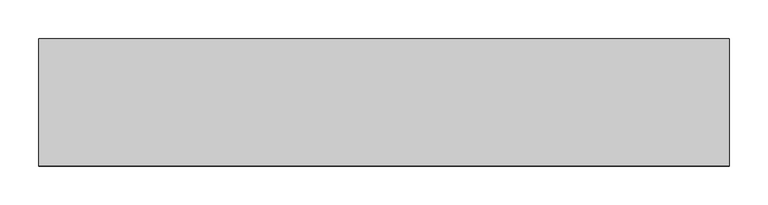
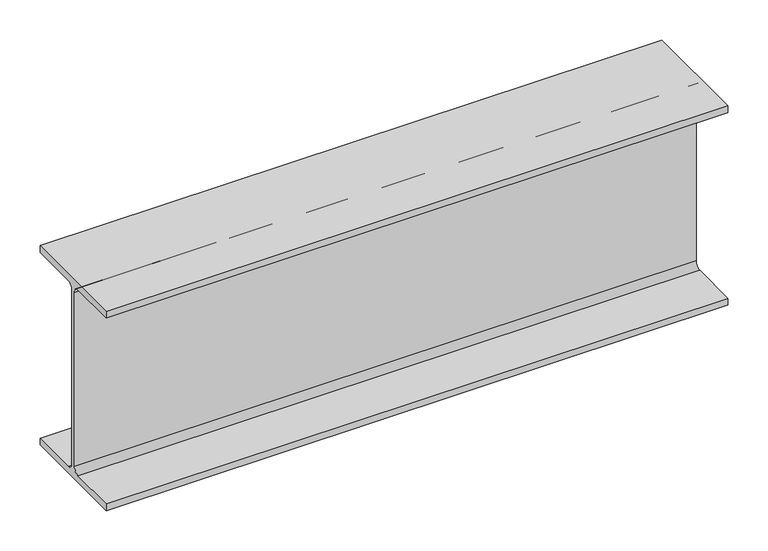
"""IFC4 building model written with IfcOpenShell, lengths in millimetres: beam geometry, Old_Steel Beam_H-KSD3502 : H_SB_ASB_H-300×150x6.5x9."""

import ifcopenshell
import ifcopenshell.guid

model = None  # the IFC model being written
_history = None  # IfcOwnerHistory: only IFC2X3 demands one
_inside = {}  # id of a spatial element -> (the spatial element, [elements in it])
_under = {}  # id of a project, library or spatial element -> (it, [spatial elements below it])
_declared = {}  # id of a project -> (the project, [libraries it declares])
_typed = {}  # id of a type object -> (the type object, [elements of that type])
_made_of = {}  # id of a material, layer set ... -> (it, [elements and type objects made of it])


def new_model(schema):
    """Start an empty IFC model of exactly this schema.

    Asked for "IFC4X3", IfcOpenShell would pick the latest addendum, in which some entities
    have other attributes; the version numbers below select the first issue.
    IFC2X3 requires an IfcOwnerHistory on every rooted entity: one is made here for all.
    """
    global model, _history
    if schema == "IFC4X3":
        model = ifcopenshell.file(schema_version=(4, 3, 0, 0))
    else:
        model = ifcopenshell.file(schema=schema)
    _inside.clear()
    _under.clear()
    _declared.clear()
    _typed.clear()
    _made_of.clear()
    _history = None
    if model.schema == "IFC2X3":
        org = make("IfcOrganization", Name="unknown")
        user = make(
            "IfcPersonAndOrganization",
            ThePerson=make("IfcPerson", FamilyName="unknown"),
            TheOrganization=org,
        )
        app = make(
            "IfcApplication",
            ApplicationDeveloper=org,
            Version="unknown",
            ApplicationFullName="unknown",
            ApplicationIdentifier="unknown",
        )
        _history = make(
            "IfcOwnerHistory",
            OwningUser=user,
            OwningApplication=app,
            ChangeAction="ADDED",
            CreationDate=0,
        )
    return model


def make(cls, **values):
    """One entity of the class cls with the attributes given. An attribute that is None is left unset."""
    return model.create_entity(
        cls, **{name: value for name, value in values.items() if value is not None}
    )


def rooted(cls, **values):
    """An entity with a GlobalId (a new one), such as an element, a storey or a relation."""
    return make(cls, GlobalId=ifcopenshell.guid.new(), OwnerHistory=_history, **values)


def si_unit(unit_type, name, prefix=None):
    """IfcSIUnit, for example si_unit("LENGTHUNIT", "METRE", prefix="MILLI")."""
    return make("IfcSIUnit", UnitType=unit_type, Prefix=prefix, Name=name)


def assignment(units):
    """IfcUnitAssignment: the units of a project."""
    return None if units is None else make("IfcUnitAssignment", Units=units)


def point(xyz):
    """IfcCartesianPoint."""
    return None if xyz is None else make("IfcCartesianPoint", Coordinates=xyz)


def direction(xyz):
    """IfcDirection."""
    return None if xyz is None else make("IfcDirection", DirectionRatios=xyz)


def frame(location, z_axis=None, x_axis=None):
    """IfcAxis2Placement3D, a coordinate frame: its origin and axes. An axis left out is left unset."""
    return make(
        "IfcAxis2Placement3D",
        Location=point(location),
        Axis=direction(z_axis),
        RefDirection=direction(x_axis),
    )


def frame_2d(location, x_axis=None):
    """IfcAxis2Placement2D, a coordinate frame in the plane: its origin and x axis."""
    return make(
        "IfcAxis2Placement2D", Location=point(location), RefDirection=direction(x_axis)
    )


def origin():
    """The frame at (0, 0, 0) with its axes left unset."""
    return frame((0.0, 0.0, 0.0))


def place(relative_to, where):
    """IfcLocalPlacement: puts the frame where relative to a parent placement (None: the world)."""
    return make(
        "IfcLocalPlacement", PlacementRelTo=relative_to, RelativePlacement=where
    )


def context(
    kind, dimensions, precision=None, world=None, true_north=None, identifier=None
):
    """IfcGeometricRepresentationContext, for example the 3D "Model" context."""
    return make(
        "IfcGeometricRepresentationContext",
        ContextIdentifier=identifier,
        ContextType=kind,
        CoordinateSpaceDimension=dimensions,
        Precision=precision,
        WorldCoordinateSystem=world,
        TrueNorth=true_north,
    )


def project(units=None, contexts=None):
    """IfcProject with its units and contexts."""
    return rooted(
        "IfcProject",
        Name="project",
        RepresentationContexts=contexts,
        UnitsInContext=assignment(units),
    )


def spatial(cls, under=None, at=None, **own):
    """A site, building, storey or space (cls), placed at a placement, below another one or the project."""
    s = rooted(cls, ObjectPlacement=at, **own)
    if under is not None:
        _under.setdefault(under.id(), (under, []))[1].append(s)
    return s


def polyline(points):
    """IfcPolyline through the points."""
    return make("IfcPolyline", Points=[point(p) for p in points])


def circle_curve(where, radius):
    """IfcCircle in the frame where."""
    return make("IfcCircle", Position=where, Radius=radius)


def trimmed(basis, trim1, trim2, sense, master):
    """IfcTrimmedCurve: the piece of a basis curve between two trims."""
    return make(
        "IfcTrimmedCurve",
        BasisCurve=basis,
        Trim1=trim1,
        Trim2=trim2,
        SenseAgreement=sense,
        MasterRepresentation=master,
    )


def segment(curve, same_sense, transition):
    """IfcCompositeCurveSegment."""
    return make(
        "IfcCompositeCurveSegment",
        Transition=transition,
        SameSense=same_sense,
        ParentCurve=curve,
    )


def composite_curve(segments, self_intersect=None):
    """IfcCompositeCurve: segments joined end to end."""
    return make("IfcCompositeCurve", Segments=segments, SelfIntersect=self_intersect)


def outline(outer, holes=None, kind="AREA"):
    """IfcArbitraryClosedProfileDef: a profile drawn as a closed curve; with holes, ...WithVoids."""
    if holes is None:
        return make("IfcArbitraryClosedProfileDef", ProfileType=kind, OuterCurve=outer)
    return make(
        "IfcArbitraryProfileDefWithVoids",
        ProfileType=kind,
        OuterCurve=outer,
        InnerCurves=holes,
    )


def extrude(swept, where, along, depth):
    """IfcExtrudedAreaSolid: the profile swept, set in the frame where, extruded along a direction by depth."""
    return make(
        "IfcExtrudedAreaSolid",
        SweptArea=swept,
        Position=where,
        ExtrudedDirection=direction(along),
        Depth=depth,
    )


def shape(context_of_items, identifier, shape_type, items):
    """IfcShapeRepresentation: the items that make up one representation, for example the "Body"."""
    return make(
        "IfcShapeRepresentation",
        ContextOfItems=context_of_items,
        RepresentationIdentifier=identifier,
        RepresentationType=shape_type,
        Items=items,
    )


def source(mapping_origin, context_of_items, identifier, shape_type, items):
    """IfcRepresentationMap: a shape defined once, which mapped items show again and again."""
    return make(
        "IfcRepresentationMap",
        MappingOrigin=mapping_origin,
        MappedRepresentation=shape(context_of_items, identifier, shape_type, items),
    )


def transform(
    local_origin,
    x_axis=None,
    y_axis=None,
    z_axis=None,
    scale=None,
    scale2=None,
    scale3=None,
    uniform=True,
):
    """IfcCartesianTransformationOperator3D, or its non-uniform kind. x_axis, y_axis, z_axis: its Axis1, 2, 3."""
    if uniform:
        return make(
            "IfcCartesianTransformationOperator3D",
            Axis1=direction(x_axis),
            Axis2=direction(y_axis),
            LocalOrigin=point(local_origin),
            Scale=scale,
            Axis3=direction(z_axis),
        )
    return make(
        "IfcCartesianTransformationOperator3DnonUniform",
        Axis1=direction(x_axis),
        Axis2=direction(y_axis),
        LocalOrigin=point(local_origin),
        Scale=scale,
        Axis3=direction(z_axis),
        Scale2=scale2,
        Scale3=scale3,
    )


def mapped(mapping_source, mapping_target):
    """IfcMappedItem: shows the shape of a source again, moved by a transform."""
    return make(
        "IfcMappedItem", MappingSource=mapping_source, MappingTarget=mapping_target
    )


def made_of(thing, what):
    """Note that an element or type object is made of a material, layer set ...; save() writes the relation."""
    if what is not None:
        _made_of.setdefault(what.id(), (what, []))[1].append(thing)
    return thing


def element(
    cls,
    number,
    at=None,
    inside=None,
    cuts=None,
    type_object=None,
    material=None,
    context=None,
    identifier="Body",
    shape_type=None,
    held_by="IfcProductDefinitionShape",
    body=None,
    shapes=None,
    **own,
):
    """One element of the class cls, such as IfcWall. Its Tag is "e" and its number.

    at: its placement. inside: the storey or other place that contains it. cuts: it is an
    opening in that element (IfcRelVoidsElement). A single representation is given by context,
    identifier, shape_type and body (its items); several are given by shapes. held_by: the class
    of the entity that holds the representations. save() writes the other relations.
    """
    e = rooted(cls, Tag="e%d" % number, ObjectPlacement=at, **own)
    if body is not None:
        shapes = [shape(context, identifier, shape_type, body)]
    if shapes is not None:
        e.Representation = make(held_by, Representations=shapes)
    if inside is not None:
        _inside.setdefault(inside.id(), (inside, []))[1].append(e)
    if cuts is not None:
        rooted(
            "IfcRelVoidsElement", RelatingBuildingElement=cuts, RelatedOpeningElement=e
        )
    if type_object is not None:
        _typed.setdefault(type_object.id(), (type_object, []))[1].append(e)
    return made_of(e, material)


def aggregate(whole, parts):
    """IfcRelAggregates: a whole, such as a stair, and the parts it consists of."""
    return rooted("IfcRelAggregates", RelatingObject=whole, RelatedObjects=parts)


def save(model, path):
    """Write the relations noted so far, then the file.

    IfcRelAggregates (storeys below a building ...), IfcRelContainedInSpatialStructure (elements
    in a storey), IfcRelDefinesByType, IfcRelAssociatesMaterial and IfcRelDeclares: one each for
    every whole, place, type object, material and project.
    """
    for whole, parts in _under.values():
        aggregate(whole, parts)
    for where, things in _inside.values():
        rooted(
            "IfcRelContainedInSpatialStructure",
            RelatedElements=things,
            RelatingStructure=where,
        )
    for kind, things in _typed.values():
        rooted("IfcRelDefinesByType", RelatedObjects=things, RelatingType=kind)
    for what, things in _made_of.values():
        rooted("IfcRelAssociatesMaterial", RelatedObjects=things, RelatingMaterial=what)
    for by, libraries in _declared.values():
        rooted("IfcRelDeclares", RelatingContext=by, RelatedDefinitions=libraries)
    model.write(path)


def beam_bd3552e1(model_context):
    return source(origin(), model_context, "Body", "SweptSolid", [
        extrude(outline(composite_curve([segment(polyline([(82.5, -141.5), (82.5, -151.7), (-82.5, -151.7), (-82.5, -141.5), (-11.9, -141.5)]), True, "CONTINUOUS"), segment(trimmed(circle_curve(frame_2d((-11.9, -132.6)), 8.9), [point((-11.9, -141.5))], [point((-3.0, -132.6))], True, "CARTESIAN"), True, "CONTINUOUS"), segment(polyline([(-3.0, -132.6), (-3.0, 132.6)]), True, "CONTINUOUS"), segment(trimmed(circle_curve(frame_2d((-11.9, 132.6)), 8.9), [point((-3.0, 132.6))], [point((-11.9, 141.5))], True, "CARTESIAN"), True, "CONTINUOUS"), segment(polyline([(-11.9, 141.5), (-82.5, 141.5), (-82.5, 151.7), (82.5, 151.7), (82.5, 141.5), (11.9, 141.5)]), True, "CONTINUOUS"), segment(trimmed(circle_curve(frame_2d((11.9, 132.6)), 8.9), [point((11.9, 141.5))], [point((3.0, 132.6))], True, "CARTESIAN"), True, "CONTINUOUS"), segment(polyline([(3.0, 132.6), (3.0, -132.6)]), True, "CONTINUOUS"), segment(trimmed(circle_curve(frame_2d((11.9, -132.6)), 8.9), [point((3.0, -132.6))], [point((11.9, -141.5))], True, "CARTESIAN"), True, "CONTINUOUS"), segment(polyline([(11.9, -141.5), (82.5, -141.5)]), True, "CONTINUOUS")], self_intersect=False)), frame((-349.8, 0.0, 0.0), z_axis=(1.0, 0.0, 0.0), x_axis=(0.0, 1.0, 0.0)), (0.0, 0.0, 1.0), 894.8),
    ])


if __name__ == "__main__":
    model = new_model("IFC4")
    model_context = context("Model", 3, world=origin())
    ifc_project = project(units=[si_unit("LENGTHUNIT", "METRE", prefix="MILLI")], contexts=[model_context])
    site = spatial("IfcSite", under=ifc_project)
    building = spatial("IfcBuilding", under=site)
    placement = place(None, origin())
    beam_shape = beam_bd3552e1(model_context)
    element("IfcBeam", 1, ObjectType="Old_Steel Beam_H-KSD3502 : H_SB_ASB_H-300×150x6.5x9", at=placement, inside=building, context=model_context, shape_type="MappedRepresentation", body=[
        mapped(beam_shape, transform((0.0, 0.0, 0.0), x_axis=(1.0, 0.0, 0.0), y_axis=(0.0, 1.0, 0.0), z_axis=(0.0, 0.0, 1.0))),
    ])
    save(model, "model.ifc")

# Revit data of these elements
# Type "Old_Steel Beam_H-KSD3502 : H_SB_ASB_H-300×150x6.5x9"
#   Width = 15.0 cm
#   Web Thickness = 0.65 cm
#   Web Fillet = 1.3 cm
#   Warping Constant = 107174.0 cm⁶
#   Torsional Moment of Inertia = 9.9539 cm⁴
#   Torsional Modulus = 1.0 cm³
#   Section Area = 46.78 cm²
#   Plastic Modulus weak axis = 105.0 cm³
#   Plastic Modulus strong axis = 542.0 cm³
#   Perimeter = 1.17 m²/m
#   Nominal Weight = 36.70 kgf/m
#   Moment of Inertia weak axis = 508.00 cm⁴
#   Moment of Inertia strong axis = 7210.00 cm⁴
#   Height = 30.0 cm
#   Flange Thickness = 0.9 cm
#   Elastic Modulus weak axis = 67.7 cm³
#   Elastic Modulus strong axis = 481.0 cm³
#   Centroid Vertical = 15.0 cm
#   Centroid Horizontal = 7.5 cm
#   Length [instance default] = 1.5240 m
#   Structural Material [instance default] = Steel, 45-345
#   Assembly Code = ""
# Element 1 (IfcBeam, "Old_Steel Beam_H-KSD3502 : H_SB_ASB_H-300×150x6.5x9")
#   Structural Material = none
# Materials
#   "Steel, 45-345": class "Metal", colour RGB 189 187 185, transparency 0, Description = "Steel 345 MPa", Cost = 0
